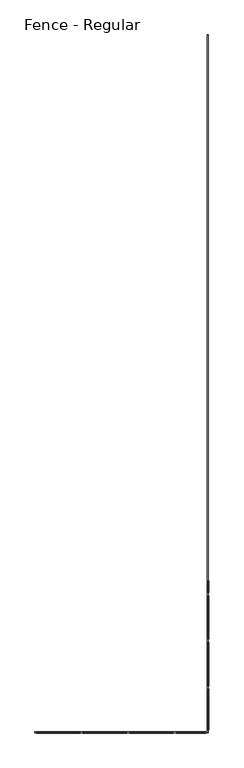
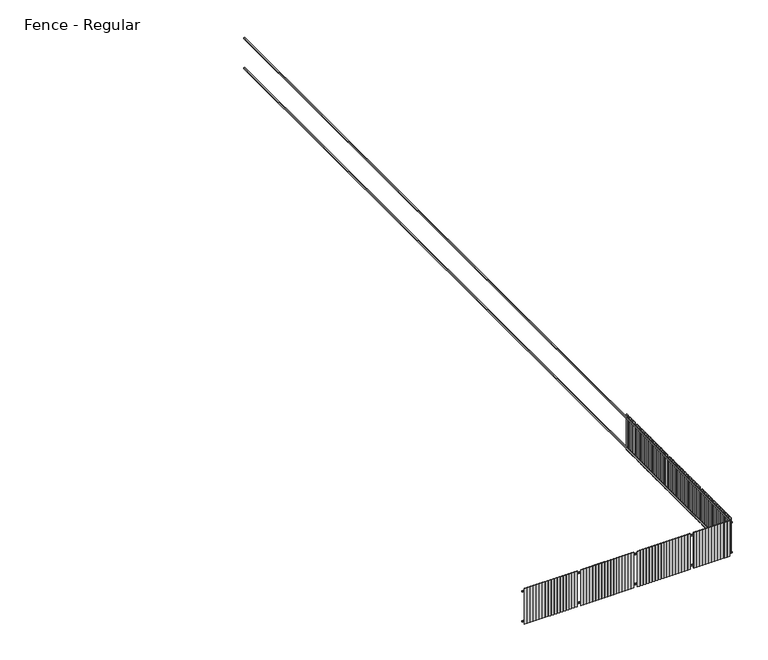
"""IFC4 building model written with IfcOpenShell, lengths in millimetres: railing geometry, Fence - Regular."""

from ifc_helpers import new_model, si_unit, origin, origin_with_axes, place, context, project, spatial, polyline, outline, extrude, faceted_brep, source, transform, mapped, element, save


def fence_regular_a554180e(model_context):
    return source(origin(), model_context, "Body", "SolidModel", [
        faceted_brep([(34556.3902986, -1683.68778, 1524.0), (34607.1902986, -1683.68778, 1524.0), (34607.1902986, -1683.68778, 1473.2), (34556.3902986, -1683.68778, 1473.2), (34556.3902986, -38139.03778, 1524.0), (34607.1902986, -38189.83778, 1524.0), (34607.1902986, -38189.83778, 1473.2), (34556.3902986, -38139.03778, 1473.2), (25533.0402986, -38139.03778, 1524.0), (25533.0402986, -38139.03778, 1473.2), (25533.0402986, -38189.83778, 1473.2), (25533.0402986, -38189.83778, 1524.0)], [[[0, 1, 2, 3]], [[1, 0, 4, 5]], [[2, 1, 5, 6]], [[3, 2, 6, 7]], [[0, 3, 7, 4]], [[8, 9, 10, 11]], [[5, 4, 8, 11]], [[6, 5, 11, 10]], [[7, 6, 10, 9]], [[4, 7, 9, 8]]]),
        faceted_brep([(34556.3902986, -1683.68778, 152.4), (34607.1902986, -1683.68778, 152.4), (34607.1902986, -1683.68778, 101.6), (34556.3902986, -1683.68778, 101.6), (34556.3902986, -38139.03778, 152.4), (34607.1902986, -38189.83778, 152.4), (34607.1902986, -38189.83778, 101.6), (34556.3902986, -38139.03778, 101.6), (25533.0402986, -38139.03778, 152.4), (25533.0402986, -38139.03778, 101.6), (25533.0402986, -38189.83778, 101.6), (25533.0402986, -38189.83778, 152.4)], [[[0, 1, 2, 3]], [[1, 0, 4, 5]], [[2, 1, 5, 6]], [[3, 2, 6, 7]], [[0, 3, 7, 4]], [[8, 9, 10, 11]], [[5, 4, 8, 11]], [[6, 5, 11, 10]], [[7, 6, 10, 9]], [[4, 7, 9, 8]]]),
        extrude(outline(polyline([(25715.3521407, -38208.88778), (25607.4021407, -38208.88778), (25607.4021407, -38189.83778), (25715.3521407, -38189.83778), (25715.3521407, -38208.88778)])), origin_with_axes(), (0.0, 0.0, 1.0), 1625.6),
        extrude(outline(polyline([(25843.6889828, -38208.88778), (25735.7389828, -38208.88778), (25735.7389828, -38189.83778), (25843.6889828, -38189.83778), (25843.6889828, -38208.88778)])), origin_with_axes(), (0.0, 0.0, 1.0), 1625.6),
        extrude(outline(polyline([(25972.0258249, -38208.88778), (25864.0758249, -38208.88778), (25864.0758249, -38189.83778), (25972.0258249, -38189.83778), (25972.0258249, -38208.88778)])), origin_with_axes(), (0.0, 0.0, 1.0), 1625.6),
        extrude(outline(polyline([(26100.3626671, -38208.88778), (25992.4126671, -38208.88778), (25992.4126671, -38189.83778), (26100.3626671, -38189.83778), (26100.3626671, -38208.88778)])), origin_with_axes(), (0.0, 0.0, 1.0), 1625.6),
        extrude(outline(polyline([(26228.6995092, -38208.88778), (26120.7495092, -38208.88778), (26120.7495092, -38189.83778), (26228.6995092, -38189.83778), (26228.6995092, -38208.88778)])), origin_with_axes(), (0.0, 0.0, 1.0), 1625.6),
        extrude(outline(polyline([(26357.0363513, -38208.88778), (26249.0863513, -38208.88778), (26249.0863513, -38189.83778), (26357.0363513, -38189.83778), (26357.0363513, -38208.88778)])), origin_with_axes(), (0.0, 0.0, 1.0), 1625.6),
        extrude(outline(polyline([(26485.3731934, -38208.88778), (26377.4231934, -38208.88778), (26377.4231934, -38189.83778), (26485.3731934, -38189.83778), (26485.3731934, -38208.88778)])), origin_with_axes(), (0.0, 0.0, 1.0), 1625.6),
        extrude(outline(polyline([(26613.7100355, -38208.88778), (26505.7600355, -38208.88778), (26505.7600355, -38189.83778), (26613.7100355, -38189.83778), (26613.7100355, -38208.88778)])), origin_with_axes(), (0.0, 0.0, 1.0), 1625.6),
        extrude(outline(polyline([(26742.0468776, -38208.88778), (26634.0968776, -38208.88778), (26634.0968776, -38189.83778), (26742.0468776, -38189.83778), (26742.0468776, -38208.88778)])), origin_with_axes(), (0.0, 0.0, 1.0), 1625.6),
        extrude(outline(polyline([(26870.3837197, -38208.88778), (26762.4337197, -38208.88778), (26762.4337197, -38189.83778), (26870.3837197, -38189.83778), (26870.3837197, -38208.88778)])), origin_with_axes(), (0.0, 0.0, 1.0), 1625.6),
        extrude(outline(polyline([(26998.7205618, -38208.88778), (26890.7705618, -38208.88778), (26890.7705618, -38189.83778), (26998.7205618, -38189.83778), (26998.7205618, -38208.88778)])), origin_with_axes(), (0.0, 0.0, 1.0), 1625.6),
        extrude(outline(polyline([(27127.0574039, -38208.88778), (27019.1074039, -38208.88778), (27019.1074039, -38189.83778), (27127.0574039, -38189.83778), (27127.0574039, -38208.88778)])), origin_with_axes(), (0.0, 0.0, 1.0), 1625.6),
        extrude(outline(polyline([(27255.394246, -38208.88778), (27147.444246, -38208.88778), (27147.444246, -38189.83778), (27255.394246, -38189.83778), (27255.394246, -38208.88778)])), origin_with_axes(), (0.0, 0.0, 1.0), 1625.6),
        extrude(outline(polyline([(27383.7310881, -38208.88778), (27275.7810881, -38208.88778), (27275.7810881, -38189.83778), (27383.7310881, -38189.83778), (27383.7310881, -38208.88778)])), origin_with_axes(), (0.0, 0.0, 1.0), 1625.6),
        extrude(outline(polyline([(27512.0679302, -38208.88778), (27404.1179302, -38208.88778), (27404.1179302, -38189.83778), (27512.0679302, -38189.83778), (27512.0679302, -38208.88778)])), origin_with_axes(), (0.0, 0.0, 1.0), 1625.6),
        extrude(outline(polyline([(27640.4047723, -38208.88778), (27532.4547723, -38208.88778), (27532.4547723, -38189.83778), (27640.4047723, -38189.83778), (27640.4047723, -38208.88778)])), origin_with_axes(), (0.0, 0.0, 1.0), 1625.6),
        extrude(outline(polyline([(27768.7416144, -38208.88778), (27660.7916144, -38208.88778), (27660.7916144, -38189.83778), (27768.7416144, -38189.83778), (27768.7416144, -38208.88778)])), origin_with_axes(), (0.0, 0.0, 1.0), 1625.6),
        extrude(outline(polyline([(27897.0784565, -38208.88778), (27789.1284565, -38208.88778), (27789.1284565, -38189.83778), (27897.0784565, -38189.83778), (27897.0784565, -38208.88778)])), origin_with_axes(), (0.0, 0.0, 1.0), 1625.6),
        extrude(outline(polyline([(28153.7521407, -38208.88778), (28045.8021407, -38208.88778), (28045.8021407, -38189.83778), (28153.7521407, -38189.83778), (28153.7521407, -38208.88778)])), origin_with_axes(), (0.0, 0.0, 1.0), 1625.6),
        extrude(outline(polyline([(28282.0889828, -38208.88778), (28174.1389828, -38208.88778), (28174.1389828, -38189.83778), (28282.0889828, -38189.83778), (28282.0889828, -38208.88778)])), origin_with_axes(), (0.0, 0.0, 1.0), 1625.6),
        extrude(outline(polyline([(28410.4258249, -38208.88778), (28302.4758249, -38208.88778), (28302.4758249, -38189.83778), (28410.4258249, -38189.83778), (28410.4258249, -38208.88778)])), origin_with_axes(), (0.0, 0.0, 1.0), 1625.6),
        extrude(outline(polyline([(28538.7626671, -38208.88778), (28430.8126671, -38208.88778), (28430.8126671, -38189.83778), (28538.7626671, -38189.83778), (28538.7626671, -38208.88778)])), origin_with_axes(), (0.0, 0.0, 1.0), 1625.6),
        extrude(outline(polyline([(28667.0995092, -38208.88778), (28559.1495092, -38208.88778), (28559.1495092, -38189.83778), (28667.0995092, -38189.83778), (28667.0995092, -38208.88778)])), origin_with_axes(), (0.0, 0.0, 1.0), 1625.6),
        extrude(outline(polyline([(28795.4363513, -38208.88778), (28687.4863513, -38208.88778), (28687.4863513, -38189.83778), (28795.4363513, -38189.83778), (28795.4363513, -38208.88778)])), origin_with_axes(), (0.0, 0.0, 1.0), 1625.6),
        extrude(outline(polyline([(28923.7731934, -38208.88778), (28815.8231934, -38208.88778), (28815.8231934, -38189.83778), (28923.7731934, -38189.83778), (28923.7731934, -38208.88778)])), origin_with_axes(), (0.0, 0.0, 1.0), 1625.6),
        extrude(outline(polyline([(29052.1100355, -38208.88778), (28944.1600355, -38208.88778), (28944.1600355, -38189.83778), (29052.1100355, -38189.83778), (29052.1100355, -38208.88778)])), origin_with_axes(), (0.0, 0.0, 1.0), 1625.6),
        extrude(outline(polyline([(29180.4468776, -38208.88778), (29072.4968776, -38208.88778), (29072.4968776, -38189.83778), (29180.4468776, -38189.83778), (29180.4468776, -38208.88778)])), origin_with_axes(), (0.0, 0.0, 1.0), 1625.6),
        extrude(outline(polyline([(29308.7837197, -38208.88778), (29200.8337197, -38208.88778), (29200.8337197, -38189.83778), (29308.7837197, -38189.83778), (29308.7837197, -38208.88778)])), origin_with_axes(), (0.0, 0.0, 1.0), 1625.6),
        extrude(outline(polyline([(29437.1205618, -38208.88778), (29329.1705618, -38208.88778), (29329.1705618, -38189.83778), (29437.1205618, -38189.83778), (29437.1205618, -38208.88778)])), origin_with_axes(), (0.0, 0.0, 1.0), 1625.6),
        extrude(outline(polyline([(29565.4574039, -38208.88778), (29457.5074039, -38208.88778), (29457.5074039, -38189.83778), (29565.4574039, -38189.83778), (29565.4574039, -38208.88778)])), origin_with_axes(), (0.0, 0.0, 1.0), 1625.6),
        extrude(outline(polyline([(29693.794246, -38208.88778), (29585.844246, -38208.88778), (29585.844246, -38189.83778), (29693.794246, -38189.83778), (29693.794246, -38208.88778)])), origin_with_axes(), (0.0, 0.0, 1.0), 1625.6),
        extrude(outline(polyline([(29822.1310881, -38208.88778), (29714.1810881, -38208.88778), (29714.1810881, -38189.83778), (29822.1310881, -38189.83778), (29822.1310881, -38208.88778)])), origin_with_axes(), (0.0, 0.0, 1.0), 1625.6),
        extrude(outline(polyline([(29950.4679302, -38208.88778), (29842.5179302, -38208.88778), (29842.5179302, -38189.83778), (29950.4679302, -38189.83778), (29950.4679302, -38208.88778)])), origin_with_axes(), (0.0, 0.0, 1.0), 1625.6),
        extrude(outline(polyline([(30078.8047723, -38208.88778), (29970.8547723, -38208.88778), (29970.8547723, -38189.83778), (30078.8047723, -38189.83778), (30078.8047723, -38208.88778)])), origin_with_axes(), (0.0, 0.0, 1.0), 1625.6),
        extrude(outline(polyline([(30207.1416144, -38208.88778), (30099.1916144, -38208.88778), (30099.1916144, -38189.83778), (30207.1416144, -38189.83778), (30207.1416144, -38208.88778)])), origin_with_axes(), (0.0, 0.0, 1.0), 1625.6),
        extrude(outline(polyline([(30335.4784565, -38208.88778), (30227.5284565, -38208.88778), (30227.5284565, -38189.83778), (30335.4784565, -38189.83778), (30335.4784565, -38208.88778)])), origin_with_axes(), (0.0, 0.0, 1.0), 1625.6),
        extrude(outline(polyline([(30592.1521407, -38208.88778), (30484.2021407, -38208.88778), (30484.2021407, -38189.83778), (30592.1521407, -38189.83778), (30592.1521407, -38208.88778)])), origin_with_axes(), (0.0, 0.0, 1.0), 1625.6),
        extrude(outline(polyline([(30720.4889828, -38208.88778), (30612.5389828, -38208.88778), (30612.5389828, -38189.83778), (30720.4889828, -38189.83778), (30720.4889828, -38208.88778)])), origin_with_axes(), (0.0, 0.0, 1.0), 1625.6),
        extrude(outline(polyline([(30848.8258249, -38208.88778), (30740.8758249, -38208.88778), (30740.8758249, -38189.83778), (30848.8258249, -38189.83778), (30848.8258249, -38208.88778)])), origin_with_axes(), (0.0, 0.0, 1.0), 1625.6),
        extrude(outline(polyline([(30977.1626671, -38208.88778), (30869.2126671, -38208.88778), (30869.2126671, -38189.83778), (30977.1626671, -38189.83778), (30977.1626671, -38208.88778)])), origin_with_axes(), (0.0, 0.0, 1.0), 1625.6),
        extrude(outline(polyline([(31105.4995092, -38208.88778), (30997.5495092, -38208.88778), (30997.5495092, -38189.83778), (31105.4995092, -38189.83778), (31105.4995092, -38208.88778)])), origin_with_axes(), (0.0, 0.0, 1.0), 1625.6),
        extrude(outline(polyline([(31233.8363513, -38208.88778), (31125.8863513, -38208.88778), (31125.8863513, -38189.83778), (31233.8363513, -38189.83778), (31233.8363513, -38208.88778)])), origin_with_axes(), (0.0, 0.0, 1.0), 1625.6),
        extrude(outline(polyline([(31362.1731934, -38208.88778), (31254.2231934, -38208.88778), (31254.2231934, -38189.83778), (31362.1731934, -38189.83778), (31362.1731934, -38208.88778)])), origin_with_axes(), (0.0, 0.0, 1.0), 1625.6),
        extrude(outline(polyline([(31490.5100355, -38208.88778), (31382.5600355, -38208.88778), (31382.5600355, -38189.83778), (31490.5100355, -38189.83778), (31490.5100355, -38208.88778)])), origin_with_axes(), (0.0, 0.0, 1.0), 1625.6),
        extrude(outline(polyline([(31618.8468776, -38208.88778), (31510.8968776, -38208.88778), (31510.8968776, -38189.83778), (31618.8468776, -38189.83778), (31618.8468776, -38208.88778)])), origin_with_axes(), (0.0, 0.0, 1.0), 1625.6),
        extrude(outline(polyline([(31747.1837197, -38208.88778), (31639.2337197, -38208.88778), (31639.2337197, -38189.83778), (31747.1837197, -38189.83778), (31747.1837197, -38208.88778)])), origin_with_axes(), (0.0, 0.0, 1.0), 1625.6),
        extrude(outline(polyline([(31875.5205618, -38208.88778), (31767.5705618, -38208.88778), (31767.5705618, -38189.83778), (31875.5205618, -38189.83778), (31875.5205618, -38208.88778)])), origin_with_axes(), (0.0, 0.0, 1.0), 1625.6),
        extrude(outline(polyline([(32003.8574039, -38208.88778), (31895.9074039, -38208.88778), (31895.9074039, -38189.83778), (32003.8574039, -38189.83778), (32003.8574039, -38208.88778)])), origin_with_axes(), (0.0, 0.0, 1.0), 1625.6),
        extrude(outline(polyline([(32132.194246, -38208.88778), (32024.244246, -38208.88778), (32024.244246, -38189.83778), (32132.194246, -38189.83778), (32132.194246, -38208.88778)])), origin_with_axes(), (0.0, 0.0, 1.0), 1625.6),
        extrude(outline(polyline([(32260.5310881, -38208.88778), (32152.5810881, -38208.88778), (32152.5810881, -38189.83778), (32260.5310881, -38189.83778), (32260.5310881, -38208.88778)])), origin_with_axes(), (0.0, 0.0, 1.0), 1625.6),
        extrude(outline(polyline([(32388.8679302, -38208.88778), (32280.9179302, -38208.88778), (32280.9179302, -38189.83778), (32388.8679302, -38189.83778), (32388.8679302, -38208.88778)])), origin_with_axes(), (0.0, 0.0, 1.0), 1625.6),
        extrude(outline(polyline([(32517.2047723, -38208.88778), (32409.2547723, -38208.88778), (32409.2547723, -38189.83778), (32517.2047723, -38189.83778), (32517.2047723, -38208.88778)])), origin_with_axes(), (0.0, 0.0, 1.0), 1625.6),
        extrude(outline(polyline([(32645.5416144, -38208.88778), (32537.5916144, -38208.88778), (32537.5916144, -38189.83778), (32645.5416144, -38189.83778), (32645.5416144, -38208.88778)])), origin_with_axes(), (0.0, 0.0, 1.0), 1625.6),
        extrude(outline(polyline([(32773.8784565, -38208.88778), (32665.9284565, -38208.88778), (32665.9284565, -38189.83778), (32773.8784565, -38189.83778), (32773.8784565, -38208.88778)])), origin_with_axes(), (0.0, 0.0, 1.0), 1625.6),
        extrude(outline(polyline([(33033.1229909, -38208.88778), (32925.1729909, -38208.88778), (32925.1729909, -38189.83778), (33033.1229909, -38189.83778), (33033.1229909, -38208.88778)])), origin_with_axes(), (0.0, 0.0, 1.0), 1625.6),
        extrude(outline(polyline([(33164.0306832, -38208.88778), (33056.0806832, -38208.88778), (33056.0806832, -38189.83778), (33164.0306832, -38189.83778), (33164.0306832, -38208.88778)])), origin_with_axes(), (0.0, 0.0, 1.0), 1625.6),
        extrude(outline(polyline([(33294.9383756, -38208.88778), (33186.9883756, -38208.88778), (33186.9883756, -38189.83778), (33294.9383756, -38189.83778), (33294.9383756, -38208.88778)])), origin_with_axes(), (0.0, 0.0, 1.0), 1625.6),
        extrude(outline(polyline([(33425.8460679, -38208.88778), (33317.8960679, -38208.88778), (33317.8960679, -38189.83778), (33425.8460679, -38189.83778), (33425.8460679, -38208.88778)])), origin_with_axes(), (0.0, 0.0, 1.0), 1625.6),
        extrude(outline(polyline([(33556.7537602, -38208.88778), (33448.8037602, -38208.88778), (33448.8037602, -38189.83778), (33556.7537602, -38189.83778), (33556.7537602, -38208.88778)])), origin_with_axes(), (0.0, 0.0, 1.0), 1625.6),
        extrude(outline(polyline([(33687.6614525, -38208.88778), (33579.7114525, -38208.88778), (33579.7114525, -38189.83778), (33687.6614525, -38189.83778), (33687.6614525, -38208.88778)])), origin_with_axes(), (0.0, 0.0, 1.0), 1625.6),
        extrude(outline(polyline([(33818.5691448, -38208.88778), (33710.6191448, -38208.88778), (33710.6191448, -38189.83778), (33818.5691448, -38189.83778), (33818.5691448, -38208.88778)])), origin_with_axes(), (0.0, 0.0, 1.0), 1625.6),
        extrude(outline(polyline([(33949.4768371, -38208.88778), (33841.5268371, -38208.88778), (33841.5268371, -38189.83778), (33949.4768371, -38189.83778), (33949.4768371, -38208.88778)])), origin_with_axes(), (0.0, 0.0, 1.0), 1625.6),
        extrude(outline(polyline([(34080.3845294, -38208.88778), (33972.4345294, -38208.88778), (33972.4345294, -38189.83778), (34080.3845294, -38189.83778), (34080.3845294, -38208.88778)])), origin_with_axes(), (0.0, 0.0, 1.0), 1625.6),
        extrude(outline(polyline([(34211.2922217, -38208.88778), (34103.3422217, -38208.88778), (34103.3422217, -38189.83778), (34211.2922217, -38189.83778), (34211.2922217, -38208.88778)])), origin_with_axes(), (0.0, 0.0, 1.0), 1625.6),
        extrude(outline(polyline([(34342.199914, -38208.88778), (34234.249914, -38208.88778), (34234.249914, -38189.83778), (34342.199914, -38189.83778), (34342.199914, -38208.88778)])), origin_with_axes(), (0.0, 0.0, 1.0), 1625.6),
        extrude(outline(polyline([(34473.1076063, -38208.88778), (34365.1576063, -38208.88778), (34365.1576063, -38189.83778), (34473.1076063, -38189.83778), (34473.1076063, -38208.88778)])), origin_with_axes(), (0.0, 0.0, 1.0), 1625.6),
        extrude(outline(polyline([(34626.2402986, -37950.3016689), (34626.2402986, -38058.2516689), (34607.1902986, -38058.2516689), (34607.1902986, -37950.3016689), (34626.2402986, -37950.3016689)])), origin_with_axes(), (0.0, 0.0, 1.0), 1625.6),
        extrude(outline(polyline([(34626.2402986, -37821.8905578), (34626.2402986, -37929.8405578), (34607.1902986, -37929.8405578), (34607.1902986, -37821.8905578), (34626.2402986, -37821.8905578)])), origin_with_axes(), (0.0, 0.0, 1.0), 1625.6),
        extrude(outline(polyline([(34626.2402986, -37693.4794467), (34626.2402986, -37801.4294467), (34607.1902986, -37801.4294467), (34607.1902986, -37693.4794467), (34626.2402986, -37693.4794467)])), origin_with_axes(), (0.0, 0.0, 1.0), 1625.6),
        extrude(outline(polyline([(34626.2402986, -37565.0683356), (34626.2402986, -37673.0183356), (34607.1902986, -37673.0183356), (34607.1902986, -37565.0683356), (34626.2402986, -37565.0683356)])), origin_with_axes(), (0.0, 0.0, 1.0), 1625.6),
        extrude(outline(polyline([(34626.2402986, -37436.6572245), (34626.2402986, -37544.6072245), (34607.1902986, -37544.6072245), (34607.1902986, -37436.6572245), (34626.2402986, -37436.6572245)])), origin_with_axes(), (0.0, 0.0, 1.0), 1625.6),
        extrude(outline(polyline([(34626.2402986, -37308.2461134), (34626.2402986, -37416.1961134), (34607.1902986, -37416.1961134), (34607.1902986, -37308.2461134), (34626.2402986, -37308.2461134)])), origin_with_axes(), (0.0, 0.0, 1.0), 1625.6),
        extrude(outline(polyline([(34626.2402986, -37179.8350023), (34626.2402986, -37287.7850023), (34607.1902986, -37287.7850023), (34607.1902986, -37179.8350023), (34626.2402986, -37179.8350023)])), origin_with_axes(), (0.0, 0.0, 1.0), 1625.6),
        extrude(outline(polyline([(34626.2402986, -37051.4238912), (34626.2402986, -37159.3738912), (34607.1902986, -37159.3738912), (34607.1902986, -37051.4238912), (34626.2402986, -37051.4238912)])), origin_with_axes(), (0.0, 0.0, 1.0), 1625.6),
        extrude(outline(polyline([(34626.2402986, -36923.01278), (34626.2402986, -37030.96278), (34607.1902986, -37030.96278), (34607.1902986, -36923.01278), (34626.2402986, -36923.01278)])), origin_with_axes(), (0.0, 0.0, 1.0), 1625.6),
        extrude(outline(polyline([(34626.2402986, -36794.6016689), (34626.2402986, -36902.5516689), (34607.1902986, -36902.5516689), (34607.1902986, -36794.6016689), (34626.2402986, -36794.6016689)])), origin_with_axes(), (0.0, 0.0, 1.0), 1625.6),
        extrude(outline(polyline([(34626.2402986, -36666.1905578), (34626.2402986, -36774.1405578), (34607.1902986, -36774.1405578), (34607.1902986, -36666.1905578), (34626.2402986, -36666.1905578)])), origin_with_axes(), (0.0, 0.0, 1.0), 1625.6),
        extrude(outline(polyline([(34626.2402986, -36537.7794467), (34626.2402986, -36645.7294467), (34607.1902986, -36645.7294467), (34607.1902986, -36537.7794467), (34626.2402986, -36537.7794467)])), origin_with_axes(), (0.0, 0.0, 1.0), 1625.6),
        extrude(outline(polyline([(34626.2402986, -36409.3683356), (34626.2402986, -36517.3183356), (34607.1902986, -36517.3183356), (34607.1902986, -36409.3683356), (34626.2402986, -36409.3683356)])), origin_with_axes(), (0.0, 0.0, 1.0), 1625.6),
        extrude(outline(polyline([(34626.2402986, -36280.9572245), (34626.2402986, -36388.9072245), (34607.1902986, -36388.9072245), (34607.1902986, -36280.9572245), (34626.2402986, -36280.9572245)])), origin_with_axes(), (0.0, 0.0, 1.0), 1625.6),
        extrude(outline(polyline([(34626.2402986, -36152.5461134), (34626.2402986, -36260.4961134), (34607.1902986, -36260.4961134), (34607.1902986, -36152.5461134), (34626.2402986, -36152.5461134)])), origin_with_axes(), (0.0, 0.0, 1.0), 1625.6),
        extrude(outline(polyline([(34626.2402986, -36024.1350023), (34626.2402986, -36132.0850023), (34607.1902986, -36132.0850023), (34607.1902986, -36024.1350023), (34626.2402986, -36024.1350023)])), origin_with_axes(), (0.0, 0.0, 1.0), 1625.6),
        extrude(outline(polyline([(34626.2402986, -35895.7238912), (34626.2402986, -36003.6738912), (34607.1902986, -36003.6738912), (34607.1902986, -35895.7238912), (34626.2402986, -35895.7238912)])), origin_with_axes(), (0.0, 0.0, 1.0), 1625.6),
        extrude(outline(polyline([(34626.2402986, -35638.9759379), (34626.2402986, -35746.9259379), (34607.1902986, -35746.9259379), (34607.1902986, -35638.9759379), (34626.2402986, -35638.9759379)])), origin_with_axes(), (0.0, 0.0, 1.0), 1625.6),
        extrude(outline(polyline([(34626.2402986, -35510.6390958), (34626.2402986, -35618.5890958), (34607.1902986, -35618.5890958), (34607.1902986, -35510.6390958), (34626.2402986, -35510.6390958)])), origin_with_axes(), (0.0, 0.0, 1.0), 1625.6),
        extrude(outline(polyline([(34626.2402986, -35382.3022537), (34626.2402986, -35490.2522537), (34607.1902986, -35490.2522537), (34607.1902986, -35382.3022537), (34626.2402986, -35382.3022537)])), origin_with_axes(), (0.0, 0.0, 1.0), 1625.6),
        extrude(outline(polyline([(34626.2402986, -35253.9654116), (34626.2402986, -35361.9154116), (34607.1902986, -35361.9154116), (34607.1902986, -35253.9654116), (34626.2402986, -35253.9654116)])), origin_with_axes(), (0.0, 0.0, 1.0), 1625.6),
        extrude(outline(polyline([(34626.2402986, -35125.6285695), (34626.2402986, -35233.5785695), (34607.1902986, -35233.5785695), (34607.1902986, -35125.6285695), (34626.2402986, -35125.6285695)])), origin_with_axes(), (0.0, 0.0, 1.0), 1625.6),
        extrude(outline(polyline([(34626.2402986, -34997.2917274), (34626.2402986, -35105.2417274), (34607.1902986, -35105.2417274), (34607.1902986, -34997.2917274), (34626.2402986, -34997.2917274)])), origin_with_axes(), (0.0, 0.0, 1.0), 1625.6),
        extrude(outline(polyline([(34626.2402986, -34868.9548853), (34626.2402986, -34976.9048853), (34607.1902986, -34976.9048853), (34607.1902986, -34868.9548853), (34626.2402986, -34868.9548853)])), origin_with_axes(), (0.0, 0.0, 1.0), 1625.6),
        extrude(outline(polyline([(34626.2402986, -34740.6180432), (34626.2402986, -34848.5680432), (34607.1902986, -34848.5680432), (34607.1902986, -34740.6180432), (34626.2402986, -34740.6180432)])), origin_with_axes(), (0.0, 0.0, 1.0), 1625.6),
        extrude(outline(polyline([(34626.2402986, -34612.2812011), (34626.2402986, -34720.2312011), (34607.1902986, -34720.2312011), (34607.1902986, -34612.2812011), (34626.2402986, -34612.2812011)])), origin_with_axes(), (0.0, 0.0, 1.0), 1625.6),
        extrude(outline(polyline([(34626.2402986, -34483.944359), (34626.2402986, -34591.894359), (34607.1902986, -34591.894359), (34607.1902986, -34483.944359), (34626.2402986, -34483.944359)])), origin_with_axes(), (0.0, 0.0, 1.0), 1625.6),
        extrude(outline(polyline([(34626.2402986, -34355.6075169), (34626.2402986, -34463.5575169), (34607.1902986, -34463.5575169), (34607.1902986, -34355.6075169), (34626.2402986, -34355.6075169)])), origin_with_axes(), (0.0, 0.0, 1.0), 1625.6),
        extrude(outline(polyline([(34626.2402986, -34227.2706748), (34626.2402986, -34335.2206748), (34607.1902986, -34335.2206748), (34607.1902986, -34227.2706748), (34626.2402986, -34227.2706748)])), origin_with_axes(), (0.0, 0.0, 1.0), 1625.6),
        extrude(outline(polyline([(34626.2402986, -34098.9338327), (34626.2402986, -34206.8838327), (34607.1902986, -34206.8838327), (34607.1902986, -34098.9338327), (34626.2402986, -34098.9338327)])), origin_with_axes(), (0.0, 0.0, 1.0), 1625.6),
        extrude(outline(polyline([(34626.2402986, -33970.5969906), (34626.2402986, -34078.5469906), (34607.1902986, -34078.5469906), (34607.1902986, -33970.5969906), (34626.2402986, -33970.5969906)])), origin_with_axes(), (0.0, 0.0, 1.0), 1625.6),
        extrude(outline(polyline([(34626.2402986, -33842.2601485), (34626.2402986, -33950.2101485), (34607.1902986, -33950.2101485), (34607.1902986, -33842.2601485), (34626.2402986, -33842.2601485)])), origin_with_axes(), (0.0, 0.0, 1.0), 1625.6),
        extrude(outline(polyline([(34626.2402986, -33713.9233064), (34626.2402986, -33821.8733064), (34607.1902986, -33821.8733064), (34607.1902986, -33713.9233064), (34626.2402986, -33713.9233064)])), origin_with_axes(), (0.0, 0.0, 1.0), 1625.6),
        extrude(outline(polyline([(34626.2402986, -33585.5864643), (34626.2402986, -33693.5364643), (34607.1902986, -33693.5364643), (34607.1902986, -33585.5864643), (34626.2402986, -33585.5864643)])), origin_with_axes(), (0.0, 0.0, 1.0), 1625.6),
        extrude(outline(polyline([(34626.2402986, -33457.2496222), (34626.2402986, -33565.1996222), (34607.1902986, -33565.1996222), (34607.1902986, -33457.2496222), (34626.2402986, -33457.2496222)])), origin_with_axes(), (0.0, 0.0, 1.0), 1625.6),
        extrude(outline(polyline([(34626.2402986, -33200.5759379), (34626.2402986, -33308.5259379), (34607.1902986, -33308.5259379), (34607.1902986, -33200.5759379), (34626.2402986, -33200.5759379)])), origin_with_axes(), (0.0, 0.0, 1.0), 1625.6),
        extrude(outline(polyline([(34626.2402986, -33072.2390958), (34626.2402986, -33180.1890958), (34607.1902986, -33180.1890958), (34607.1902986, -33072.2390958), (34626.2402986, -33072.2390958)])), origin_with_axes(), (0.0, 0.0, 1.0), 1625.6),
        extrude(outline(polyline([(34626.2402986, -32943.9022537), (34626.2402986, -33051.8522537), (34607.1902986, -33051.8522537), (34607.1902986, -32943.9022537), (34626.2402986, -32943.9022537)])), origin_with_axes(), (0.0, 0.0, 1.0), 1625.6),
        extrude(outline(polyline([(34626.2402986, -32815.5654116), (34626.2402986, -32923.5154116), (34607.1902986, -32923.5154116), (34607.1902986, -32815.5654116), (34626.2402986, -32815.5654116)])), origin_with_axes(), (0.0, 0.0, 1.0), 1625.6),
        extrude(outline(polyline([(34626.2402986, -32687.2285695), (34626.2402986, -32795.1785695), (34607.1902986, -32795.1785695), (34607.1902986, -32687.2285695), (34626.2402986, -32687.2285695)])), origin_with_axes(), (0.0, 0.0, 1.0), 1625.6),
        extrude(outline(polyline([(34626.2402986, -32558.8917274), (34626.2402986, -32666.8417274), (34607.1902986, -32666.8417274), (34607.1902986, -32558.8917274), (34626.2402986, -32558.8917274)])), origin_with_axes(), (0.0, 0.0, 1.0), 1625.6),
        extrude(outline(polyline([(34626.2402986, -32430.5548853), (34626.2402986, -32538.5048853), (34607.1902986, -32538.5048853), (34607.1902986, -32430.5548853), (34626.2402986, -32430.5548853)])), origin_with_axes(), (0.0, 0.0, 1.0), 1625.6),
        extrude(outline(polyline([(34626.2402986, -32302.2180432), (34626.2402986, -32410.1680432), (34607.1902986, -32410.1680432), (34607.1902986, -32302.2180432), (34626.2402986, -32302.2180432)])), origin_with_axes(), (0.0, 0.0, 1.0), 1625.6),
        extrude(outline(polyline([(34626.2402986, -32173.8812011), (34626.2402986, -32281.8312011), (34607.1902986, -32281.8312011), (34607.1902986, -32173.8812011), (34626.2402986, -32173.8812011)])), origin_with_axes(), (0.0, 0.0, 1.0), 1625.6),
        extrude(outline(polyline([(34626.2402986, -32045.544359), (34626.2402986, -32153.494359), (34607.1902986, -32153.494359), (34607.1902986, -32045.544359), (34626.2402986, -32045.544359)])), origin_with_axes(), (0.0, 0.0, 1.0), 1625.6),
        extrude(outline(polyline([(34626.2402986, -31917.2075169), (34626.2402986, -32025.1575169), (34607.1902986, -32025.1575169), (34607.1902986, -31917.2075169), (34626.2402986, -31917.2075169)])), origin_with_axes(), (0.0, 0.0, 1.0), 1625.6),
        extrude(outline(polyline([(34626.2402986, -31788.8706748), (34626.2402986, -31896.8206748), (34607.1902986, -31896.8206748), (34607.1902986, -31788.8706748), (34626.2402986, -31788.8706748)])), origin_with_axes(), (0.0, 0.0, 1.0), 1625.6),
        extrude(outline(polyline([(34626.2402986, -31660.5338327), (34626.2402986, -31768.4838327), (34607.1902986, -31768.4838327), (34607.1902986, -31660.5338327), (34626.2402986, -31660.5338327)])), origin_with_axes(), (0.0, 0.0, 1.0), 1625.6),
        extrude(outline(polyline([(34626.2402986, -31532.1969906), (34626.2402986, -31640.1469906), (34607.1902986, -31640.1469906), (34607.1902986, -31532.1969906), (34626.2402986, -31532.1969906)])), origin_with_axes(), (0.0, 0.0, 1.0), 1625.6),
        extrude(outline(polyline([(34626.2402986, -31403.8601485), (34626.2402986, -31511.8101485), (34607.1902986, -31511.8101485), (34607.1902986, -31403.8601485), (34626.2402986, -31403.8601485)])), origin_with_axes(), (0.0, 0.0, 1.0), 1625.6),
        extrude(outline(polyline([(34626.2402986, -31275.5233064), (34626.2402986, -31383.4733064), (34607.1902986, -31383.4733064), (34607.1902986, -31275.5233064), (34626.2402986, -31275.5233064)])), origin_with_axes(), (0.0, 0.0, 1.0), 1625.6),
        extrude(outline(polyline([(34626.2402986, -31147.1864643), (34626.2402986, -31255.1364643), (34607.1902986, -31255.1364643), (34607.1902986, -31147.1864643), (34626.2402986, -31147.1864643)])), origin_with_axes(), (0.0, 0.0, 1.0), 1625.6),
        extrude(outline(polyline([(34626.2402986, -31018.8496222), (34626.2402986, -31126.7996222), (34607.1902986, -31126.7996222), (34607.1902986, -31018.8496222), (34626.2402986, -31018.8496222)])), origin_with_axes(), (0.0, 0.0, 1.0), 1625.6),
        extrude(outline(polyline([(34626.2402986, -30762.1759379), (34626.2402986, -30870.1259379), (34607.1902986, -30870.1259379), (34607.1902986, -30762.1759379), (34626.2402986, -30762.1759379)])), origin_with_axes(), (0.0, 0.0, 1.0), 1625.6),
        extrude(outline(polyline([(34626.2402986, -30633.8390958), (34626.2402986, -30741.7890958), (34607.1902986, -30741.7890958), (34607.1902986, -30633.8390958), (34626.2402986, -30633.8390958)])), origin_with_axes(), (0.0, 0.0, 1.0), 1625.6),
        extrude(outline(polyline([(34626.2402986, -30505.5022537), (34626.2402986, -30613.4522537), (34607.1902986, -30613.4522537), (34607.1902986, -30505.5022537), (34626.2402986, -30505.5022537)])), origin_with_axes(), (0.0, 0.0, 1.0), 1625.6),
        extrude(outline(polyline([(34626.2402986, -30377.1654116), (34626.2402986, -30485.1154116), (34607.1902986, -30485.1154116), (34607.1902986, -30377.1654116), (34626.2402986, -30377.1654116)])), origin_with_axes(), (0.0, 0.0, 1.0), 1625.6),
        extrude(outline(polyline([(34626.2402986, -30248.8285695), (34626.2402986, -30356.7785695), (34607.1902986, -30356.7785695), (34607.1902986, -30248.8285695), (34626.2402986, -30248.8285695)])), origin_with_axes(), (0.0, 0.0, 1.0), 1625.6),
    ])


if __name__ == "__main__":
    model = new_model("IFC4")
    model_context = context("Model", 3, world=origin())
    ifc_project = project(units=[si_unit("LENGTHUNIT", "METRE", prefix="MILLI")], contexts=[model_context])
    site = spatial("IfcSite", under=ifc_project)
    building = spatial("IfcBuilding", under=site)
    placement = place(None, origin())
    fence_regular_shape = fence_regular_a554180e(model_context)
    element("IfcRailing", 1, ObjectType="Fence - Regular", at=placement, inside=building, context=model_context, shape_type="MappedRepresentation", body=[
        mapped(fence_regular_shape, transform((0.0, 0.0, 0.0), x_axis=(1.0, 0.0, 0.0), y_axis=(0.0, 1.0, 0.0), z_axis=(0.0, 0.0, 1.0))),
    ])
    save(model, "model.ifc")

# Revit data of these elements
# Element 1 (IfcRailing, "Fence - Regular")
#   Materials on its faces: "6FT HIGH CEDAR PRIVACY FENCE (SEE DETAIL 3A/A500)"
# Materials
#   "6FT HIGH CEDAR PRIVACY FENCE (SEE DETAIL 3A/A500)": class "Wood", colour RGB 146 120 101, transparency 0, Cost = 0
